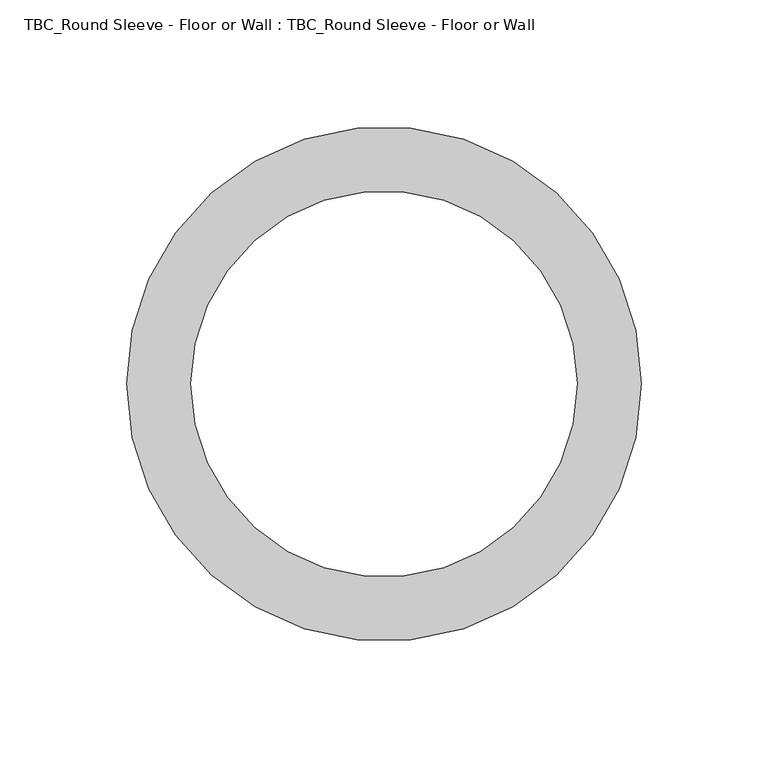
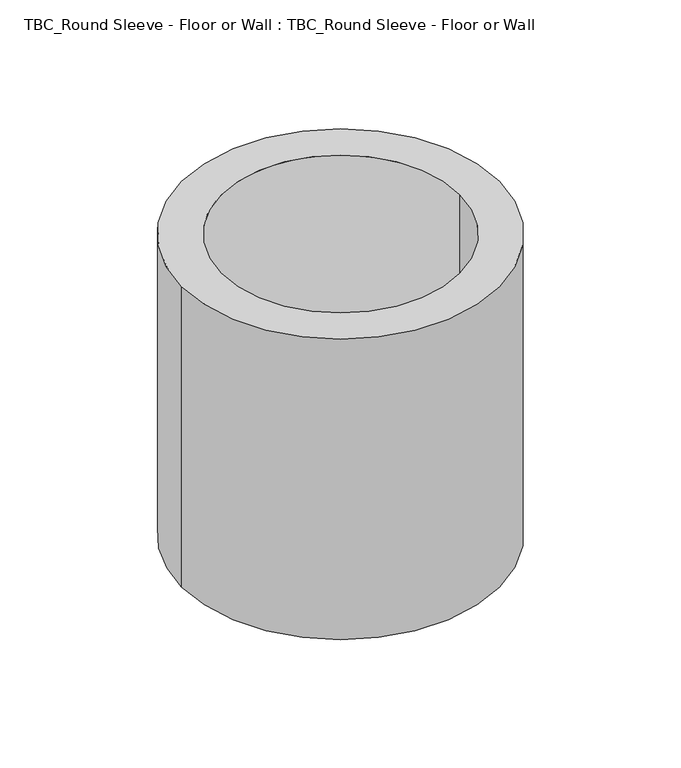
"""IFC4 building model written with IfcOpenShell, lengths in millimetres: proxy geometry, TBC_Round Sleeve - Floor or Wall : TBC_Round Sleeve - Floor or Wall."""

from ifc_helpers import new_model, si_unit, point, frame, origin, origin_2d, place, context, project, spatial, circle_curve, trimmed, segment, composite_curve, outline, extrude, source, transform, mapped, element, save


def tbc_round_sleeve_floor_or_wall_tbc_round_sleeve_floor_or_d9b5ee57(model_context):
    return source(origin(), model_context, "Body", "SweptSolid", [
        extrude(outline(composite_curve([segment(trimmed(circle_curve(origin_2d(), 101.6), [point((-101.6, 0.0))], [point((101.6, 0.0))], False, "CARTESIAN"), True, "CONTINUOUS"), segment(trimmed(circle_curve(origin_2d(), 101.6), [point((101.6, 0.0))], [point((-101.6, 0.0))], False, "CARTESIAN"), True, "CONTINUOUS")], self_intersect=False), holes=[composite_curve([segment(trimmed(circle_curve(origin_2d(), 76.2), [point((-76.2, 0.0))], [point((76.2, 0.0))], True, "CARTESIAN"), True, "CONTINUOUS"), segment(trimmed(circle_curve(origin_2d(), 76.2), [point((76.2, 0.0))], [point((-76.2, 0.0))], True, "CARTESIAN"), True, "CONTINUOUS")], self_intersect=False)]), frame((0.0, 0.0, -203.2), z_axis=(0.0, 0.0, 1.0), x_axis=(1.0, 0.0, 0.0)), (0.0, 0.0, 1.0), 203.2),
    ])


if __name__ == "__main__":
    model = new_model("IFC4")
    model_context = context("Model", 3, world=origin())
    ifc_project = project(units=[si_unit("LENGTHUNIT", "METRE", prefix="MILLI")], contexts=[model_context])
    site = spatial("IfcSite", under=ifc_project)
    building = spatial("IfcBuilding", under=site)
    placement = place(None, origin())
    tbc_round_sleeve_floor_or_wall_tbc_round_sleeve_floor_or_shape = tbc_round_sleeve_floor_or_wall_tbc_round_sleeve_floor_or_d9b5ee57(model_context)
    element("IfcBuildingElementProxy", 1, Name="TBC_Round Sleeve - Floor or Wall : TBC_Round Sleeve - Floor or Wall", ObjectType="TBC_Round Sleeve - Floor or Wall : TBC_Round Sleeve - Floor or Wall", at=placement, inside=building, context=model_context, shape_type="MappedRepresentation", body=[
        mapped(tbc_round_sleeve_floor_or_wall_tbc_round_sleeve_floor_or_shape, transform((0.0, 0.0, 0.0), x_axis=(1.0, 0.0, 0.0), y_axis=(0.0, 1.0, 0.0), z_axis=(0.0, 0.0, 1.0))),
    ])
    save(model, "model.ifc")

# Revit data of these elements
# Type "TBC_Round Sleeve - Floor or Wall : TBC_Round Sleeve - Floor or Wall"
#   Tag Dimension [instance default] = ""
#   MEP Type [instance default] = ""
#   MEP Element [instance default] = ""
#   MEP Category [instance default] = ""
#   Host Element Type [instance default] = ""
#   Host Element Id [instance default] = ""
#   Host Element Category [instance default] = ""
#   Control Line Y [instance default] = ""
#   Control Line X [instance default] = ""
#   Sleeve Radius [instance default] = 1' - 0"
#   Sleeve Edge [instance default] = 1' - 2"
#   Sleeve Depth [instance default] = 3' - 0"
#   Distance Y [instance default] = 0' - 0"
#   Distance X [instance default] = 0' - 0"
#   Default Elevation = 0
# Element 1 (IfcBuildingElementProxy, "TBC_Round Sleeve - Floor or Wall : TBC_Round Sleeve - Floor or Wall")
#   Tag Dimension = "8\"ø"
#   MEP Type = "PLG-G"
#   MEP Element = "904461"
#   MEP Category = "Pipe"
#   Host Element Type = "8\" Plank"
#   Host Element Id = "529506"
#   Host Element Category = "Floors"
#   Sleeve Radius = 0' - 6"
#   Sleeve Edge = 0' - 8"
#   Sleeve Depth = 0' - 8"
